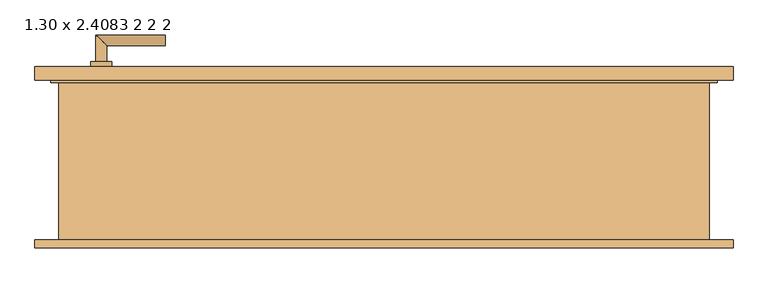
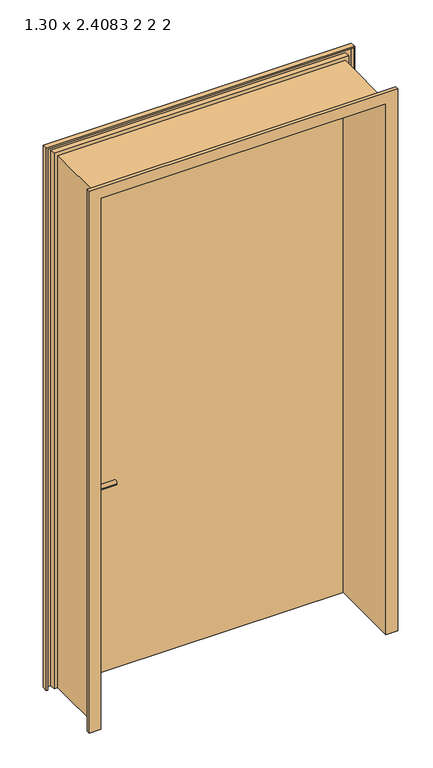
"""IFC4 building model written with IfcOpenShell, lengths in millimetres: door geometry, Drehflügel 1-flg - Stahlzarge : 1.30 x 2.4083 2 2 2."""

from ifc_helpers import new_model, si_unit, point, frame, frame_2d, origin, place, context, project, spatial, polyline, circle_curve, ellipse_curve, trimmed, segment, composite_curve, outline, extrude, faceted_brep, source, transform, mapped, element, save
from ifc_brep_helpers import plane_surface, cylinder_surface, advanced_brep


def door_1_30_x_2_4083_2_2_2_ebc270b9(model_context):
    return source(origin(), model_context, "Body", "SolidModel", [
        advanced_brep(
        [(-540.0, 139.4346141, 915.0), (-520.0, 139.4346141, 915.0), (-540.0, 69.4346141, 915.0), (-520.0, 89.4346141, 915.0), (-410.0, 69.4346141, 915.0), (-410.0, 89.4346141, 915.0)],
        [
            (0, 1, circle_curve(frame((-530.0, 139.4346141, 915.0), z_axis=(0.0, 1.0, 0.0), x_axis=(1.0, 0.0, 0.0)), 10.0)),
            (1, 0, circle_curve(frame((-530.0, 139.4346141, 915.0), z_axis=(0.0, 1.0, 0.0), x_axis=(1.0, 0.0, 0.0)), 10.0)),
            (0, 2),
            (2, 3, ellipse_curve(frame((-530.0, 79.4346141, 915.0), z_axis=(-0.7071067811865385, 0.7071067811865565, 0.0), x_axis=(0.7071067811865563, 0.7071067811865386, 0.0)), 14.1421356, 10.0)),
            (3, 1),
            (3, 2, ellipse_curve(frame((-530.0, 79.4346141, 915.0), z_axis=(-0.7071067811865385, 0.7071067811865565, 0.0), x_axis=(0.7071067811865563, 0.7071067811865386, 0.0)), 14.1421356, 10.0)),
            (4, 5, circle_curve(frame((-410.0, 79.4346141, 915.0), z_axis=(1.0, 0.0, 0.0), x_axis=(0.0, 1.0, 0.0)), 10.0)),
            (5, 4, circle_curve(frame((-410.0, 79.4346141, 915.0), z_axis=(1.0, 0.0, 0.0), x_axis=(0.0, 1.0, 0.0)), 10.0)),
            (2, 4),
            (5, 3),
        ],
        [
            plane_surface(frame((-530.0, 139.4346141, -372.7526403), z_axis=(0.0, 1.0, 0.0), x_axis=(0.0, 0.0, 1.0))),
            cylinder_surface(frame((-530.0, 139.4346141, 915.0), z_axis=(0.0, 1.0, 0.0), x_axis=(1.0, 0.0, 0.0)), 10.0),
            plane_surface(frame((-410.0, 79.4346141, -372.7526403), z_axis=(1.0, 0.0, 0.0), x_axis=(0.0, 0.0, 1.0))),
            cylinder_surface(frame((-530.0, 79.4346141, 915.0), z_axis=(-1.0, 0.0, 0.0), x_axis=(0.0, 1.0, 0.0)), 10.0),
        ],
        [
            (0, [[1, 2]]),
            (1, [[-1, 3, 4, 5]]),
            (1, [[-2, -5, 6, -3]]),
            (2, [[7, 8]]),
            (3, [[-4, 9, -8, 10]]),
            (3, [[-6, -10, -7, -9]]),
        ],
    ),
        advanced_brep(
        [(-520.0, 199.4346141, 915.0), (-540.0, 199.4346141, 915.0), (-520.0, 229.4346141, 915.0), (-540.0, 249.4346141, 915.0), (-410.0, 229.4346141, 915.0), (-410.0, 249.4346141, 915.0)],
        [
            (0, 1, circle_curve(frame((-530.0, 199.4346141, 915.0), z_axis=(0.0, -1.0, 0.0), x_axis=(-1.0, 0.0, 0.0)), 10.0)),
            (1, 0, circle_curve(frame((-530.0, 199.4346141, 915.0), z_axis=(0.0, -1.0, 0.0), x_axis=(-1.0, 0.0, 0.0)), 10.0)),
            (0, 2),
            (2, 3, ellipse_curve(frame((-530.0, 239.4346141, 915.0), z_axis=(-0.7071067811865475, -0.7071067811865475, 0.0), x_axis=(0.7071067811865474, -0.7071067811865476, 0.0)), 14.1421356, 10.0)),
            (3, 1),
            (3, 2, ellipse_curve(frame((-530.0, 239.4346141, 915.0), z_axis=(-0.7071067811865475, -0.7071067811865475, 0.0), x_axis=(0.7071067811865474, -0.7071067811865476, 0.0)), 14.1421356, 10.0)),
            (4, 5, circle_curve(frame((-410.0, 239.4346141, 915.0), z_axis=(1.0, 0.0, 0.0), x_axis=(0.0, 1.0, 0.0)), 10.0)),
            (5, 4, circle_curve(frame((-410.0, 239.4346141, 915.0), z_axis=(1.0, 0.0, 0.0), x_axis=(0.0, 1.0, 0.0)), 10.0)),
            (2, 4),
            (5, 3),
        ],
        [
            plane_surface(frame((-530.0, 199.4346141, -372.7526403), z_axis=(0.0, -1.0, 0.0), x_axis=(0.0, 0.0, 1.0))),
            cylinder_surface(frame((-530.0, 199.4346141, 915.0), z_axis=(0.0, -1.0, 0.0), x_axis=(-1.0, 0.0, 0.0)), 10.0),
            plane_surface(frame((-410.0, 239.4346141, -372.7526403), z_axis=(1.0, 0.0, 0.0), x_axis=(0.0, 0.0, 1.0))),
            cylinder_surface(frame((-530.0, 239.4346141, 915.0), z_axis=(-1.0, 0.0, 0.0), x_axis=(0.0, 1.0, 0.0)), 10.0),
        ],
        [
            (0, [[1, 2]]),
            (1, [[-1, 3, 4, 5]]),
            (1, [[-2, -5, 6, -3]]),
            (2, [[7, 8]]),
            (3, [[-4, 9, -8, 10]]),
            (3, [[-6, -10, -7, -9]]),
        ],
    ),
        extrude(outline(composite_curve([segment(trimmed(circle_curve(frame_2d((915.0, -530.0)), 20.0), [point((915.0, -550.0))], [point((915.0, -510.0))], False, "CARTESIAN"), True, "CONTINUOUS"), segment(trimmed(circle_curve(frame_2d((915.0, -530.0)), 20.0), [point((915.0, -510.0))], [point((915.0, -550.0))], False, "CARTESIAN"), True, "CONTINUOUS")], self_intersect=False)), frame((0.0, 129.4346141, 0.0), z_axis=(0.0, 1.0, 0.0), x_axis=(0.0, 0.0, 1.0)), (0.0, 0.0, 1.0), 10.0),
        extrude(outline(composite_curve([segment(trimmed(circle_curve(frame_2d((915.0, -530.0)), 20.0), [point((915.0, -550.0))], [point((915.0, -510.0))], False, "CARTESIAN"), True, "CONTINUOUS"), segment(trimmed(circle_curve(frame_2d((915.0, -530.0)), 20.0), [point((915.0, -510.0))], [point((915.0, -550.0))], False, "CARTESIAN"), True, "CONTINUOUS")], self_intersect=False)), frame((0.0, 189.4346141, 0.0), z_axis=(0.0, 1.0, 0.0), x_axis=(0.0, 0.0, 1.0)), (0.0, 0.0, 1.0), 10.0),
        extrude(outline(polyline([(620.0, 164.4346141), (-620.0, 164.4346141), (-620.0, 189.4346141), (620.0, 189.4346141), (620.0, 164.4346141)])), frame((0.0, 0.0, 15.0), z_axis=(0.0, 0.0, 1.0), x_axis=(1.0, 0.0, 0.0)), (0.0, 0.0, 1.0), 2398.3),
        faceted_brep([(654.4603207, -150.5653859, 15.0), (605.0, -150.5653859, 15.0), (605.0, 164.4346141, 15.0), (620.0, 164.4346141, 15.0), (620.0, 189.4346141, 15.0), (654.4603207, 189.4346141, 15.0), (654.4603207, 164.4346141, 15.0), (649.4603207, 164.4346141, 15.0), (649.4603207, 184.4346141, 15.0), (625.0, 184.4346141, 15.0), (625.0, 159.4346141, 15.0), (610.0, 159.4346141, 15.0), (610.0, -145.5653859, 15.0), (649.4603207, -145.5653859, 15.0), (649.4603207, -135.5653859, 15.0), (654.4603207, -135.5653859, 15.0), (654.4603207, -150.5653859, 2447.7603207), (-654.4603207, -150.5653859, 2447.7603207), (-654.4603207, -150.5653859, 15.0), (-605.0, -150.5653859, 15.0), (-605.0, -150.5653859, 2398.3), (605.0, -150.5653859, 2398.3), (605.0, 164.4346141, 2398.3), (-605.0, 164.4346141, 2398.3), (-605.0, 164.4346141, 15.0), (-620.0, 164.4346141, 15.0), (-620.0, 164.4346141, 2413.3), (620.0, 164.4346141, 2413.3), (620.0, 189.4346141, 2413.3), (-620.0, 189.4346141, 2413.3), (-620.0, 189.4346141, 15.0), (-654.4603207, 189.4346141, 15.0), (-654.4603207, 189.4346141, 2447.7603207), (654.4603207, 189.4346141, 2447.7603207), (654.4603207, 164.4346141, 2447.7603207), (-654.4603207, 164.4346141, 2447.7603207), (-654.4603207, 164.4346141, 15.0), (-649.4603207, 164.4346141, 15.0), (-649.4603207, 164.4346141, 2442.7603207), (649.4603207, 164.4346141, 2442.7603207), (649.4603207, 184.4346141, 2442.7603207), (-649.4603207, 184.4346141, 2442.7603207), (-649.4603207, 184.4346141, 15.0), (-625.0, 184.4346141, 15.0), (-625.0, 184.4346141, 2418.3), (625.0, 184.4346141, 2418.3), (625.0, 159.4346141, 2418.3), (-625.0, 159.4346141, 2418.3), (-625.0, 159.4346141, 15.0), (-610.0, 159.4346141, 15.0), (-610.0, 159.4346141, 2403.3), (610.0, 159.4346141, 2403.3), (610.0, -145.5653859, 2403.3), (-610.0, -145.5653859, 2403.3), (-610.0, -145.5653859, 15.0), (-649.4603207, -145.5653859, 15.0), (-649.4603207, -145.5653859, 2442.7603207), (649.4603207, -145.5653859, 2442.7603207), (649.4603207, -135.5653859, 2442.7603207), (-649.4603207, -135.5653859, 2442.7603207), (-649.4603207, -135.5653859, 15.0), (-654.4603207, -135.5653859, 15.0), (-654.4603207, -135.5653859, 2447.7603207), (654.4603207, -135.5653859, 2447.7603207)], [[[0, 1, 2, 3, 4, 5, 6, 7, 8, 9, 10, 11, 12, 13, 14, 15]], [[1, 0, 16, 17, 18, 19, 20, 21]], [[2, 1, 21, 22]], [[3, 2, 22, 23, 24, 25, 26, 27]], [[4, 3, 27, 28]], [[5, 4, 28, 29, 30, 31, 32, 33]], [[6, 5, 33, 34]], [[7, 6, 34, 35, 36, 37, 38, 39]], [[8, 7, 39, 40]], [[9, 8, 40, 41, 42, 43, 44, 45]], [[10, 9, 45, 46]], [[11, 10, 46, 47, 48, 49, 50, 51]], [[12, 11, 51, 52]], [[13, 12, 52, 53, 54, 55, 56, 57]], [[14, 13, 57, 58]], [[15, 14, 58, 59, 60, 61, 62, 63]], [[0, 15, 63, 16]], [[17, 62, 61, 18]], [[18, 61, 60, 55, 54, 49, 48, 43, 42, 37, 36, 31, 30, 25, 24, 19]], [[23, 20, 19, 24]], [[29, 26, 25, 30]], [[35, 32, 31, 36]], [[41, 38, 37, 42]], [[47, 44, 43, 48]], [[53, 50, 49, 54]], [[59, 56, 55, 60]], [[22, 21, 20, 23]], [[28, 27, 26, 29]], [[34, 33, 32, 35]], [[40, 39, 38, 41]], [[46, 45, 44, 47]], [[52, 51, 50, 53]], [[58, 57, 56, 59]], [[16, 63, 62, 17]]]),
    ])


if __name__ == "__main__":
    model = new_model("IFC4")
    model_context = context("Model", 3, world=origin())
    ifc_project = project(units=[si_unit("LENGTHUNIT", "METRE", prefix="MILLI")], contexts=[model_context])
    site = spatial("IfcSite", under=ifc_project)
    building = spatial("IfcBuilding", under=site)
    placement = place(None, origin())
    door_1_30_x_2_4083_2_2_2_shape = door_1_30_x_2_4083_2_2_2_ebc270b9(model_context)
    element("IfcDoor", 1, ObjectType="Drehflügel 1-flg - Stahlzarge : 1.30 x 2.4083 2 2 2", at=placement, inside=building, context=model_context, shape_type="MappedRepresentation", body=[
        mapped(door_1_30_x_2_4083_2_2_2_shape, transform((0.0, 0.0, 0.0), x_axis=(1.0, 0.0, 0.0), y_axis=(0.0, 1.0, 0.0), z_axis=(0.0, 0.0, 1.0))),
    ])
    save(model, "model.ifc")

# Revit data of these elements
# Type "Drehflügel 1-flg - Stahlzarge : 1.30 x 2.4083 2 2 2"
#   Type Mark = "26"
#   Operation = "SingleSwingRight"
#   Keynote = "16.03"
#   Analytic Construction = "Metall"
#   Thermal Resistance (R) = 0.270117 (m²·K)/W
#   Heat Transfer Coefficient (U) = 3.7021 W/(m²·K)
#   Rough Width = 1.260 m
#   Rough Height [instance default] = 2.5083 m
#   Höhe Türgriff [instance default] = 0.900 m
#   Height = 2.4083 m
#   Fußbodenaufbau [instance default] = 0.100 m
#   Width = 1.260 m
#   Sichtbarkeit Sturzlinien [instance default] = yes
#   Türgriff auswählen [instance default] = element 221079
#   Türgriff [instance default] = none
#   Türflügel [instance default] = none
#   Rahmen/Pfosten [instance default] = Metall - Lackiert - Grau
#   Visual Light Transmittance = 0
#   Solar Heat Gain Coefficient = 0
#   Function = (empty or 0)
#   Wall Closure = (empty or 0)
# Element 1 (IfcDoor, "Drehflügel 1-flg - Stahlzarge : 1.30 x 2.4083 2 2 2")
#   Rough Height = 2.4233 m
#   Fußbodenaufbau = 0.015 m
#   Materials on its faces: "Metall - Lackiert - Grau", "Metall - Chrom", "Holz - Birke"
# Materials
#   "Metall - Lackiert - Grau": class "Farbe 1", colour RGB 98 98 98, transparency 0, Cost = 0
#   "Metall - Chrom": class "Metall", colour RGB 247 247 247, transparency 0, Cost = 0
#   "Holz - Birke": class "Holz", colour RGB 213 164 103, transparency 0, Cost = 0
